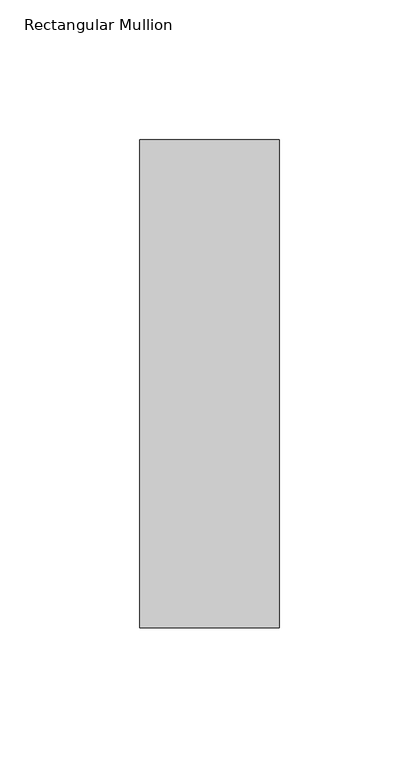
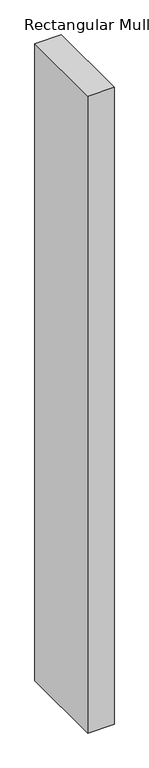
"""IFC4 building model written with IfcOpenShell, lengths in millimetres: member geometry, Rectangular Mullion : WWm-50x175-50mmOffset."""

from ifc_helpers import new_model, si_unit, frame, origin, place, context, project, spatial, polyline, outline, extrude, source, transform, mapped, element, save


def rectangular_mullion_d2ddfd06(model_context):
    return source(origin(), model_context, "Body", "SweptSolid", [
        extrude(outline(polyline([(0.0, 87.5), (0.0, -87.5), (-50.0, -87.5), (-50.0, 87.5), (0.0, 87.5)])), frame((0.0, 0.0, -1285.3388603), z_axis=(0.0, 0.0, 1.0), x_axis=(1.0, 0.0, 0.0)), (0.0, 0.0, 1.0), 1285.3388603),
    ])


if __name__ == "__main__":
    model = new_model("IFC4")
    model_context = context("Model", 3, world=origin())
    ifc_project = project(units=[si_unit("LENGTHUNIT", "METRE", prefix="MILLI")], contexts=[model_context])
    site = spatial("IfcSite", under=ifc_project)
    building = spatial("IfcBuilding", under=site)
    placement = place(None, origin())
    rectangular_mullion_shape = rectangular_mullion_d2ddfd06(model_context)
    element("IfcMember", 1, ObjectType="Rectangular Mullion : WWm-50x175-50mmOffset", at=placement, inside=building, context=model_context, shape_type="MappedRepresentation", body=[
        mapped(rectangular_mullion_shape, transform((0.0, 0.0, 0.0), x_axis=(1.0, 0.0, 0.0), y_axis=(0.0, 1.0, 0.0), z_axis=(0.0, 0.0, 1.0))),
    ])
    save(model, "model.ifc")

# Revit data of these elements
# Type "Rectangular Mullion : WWm-50x175-50mmOffset"
#   built-in parameter 1007304 = 0.574147 (stored number, unit not read)
#   built-in parameter 1007301 = 0.082021 (stored number, unit not read)
#   built-in parameter 1007300 = 0.082021 (stored number, unit not read)
# Element 1 (IfcMember, "Rectangular Mullion : WWm-50x175-50mmOffset")
#   Materials on its faces: "WW-EC-RGB-Mullion"
# Materials
#   "WW-EC-RGB-Mullion": class "Generic", colour RGB 255 255 255, transparency 0, Comments = "If region requests black mullions, switch asset color to RGB 25-25-25", Description = "Generic Color", Cost = 0
